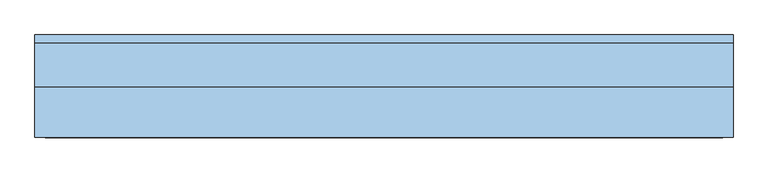
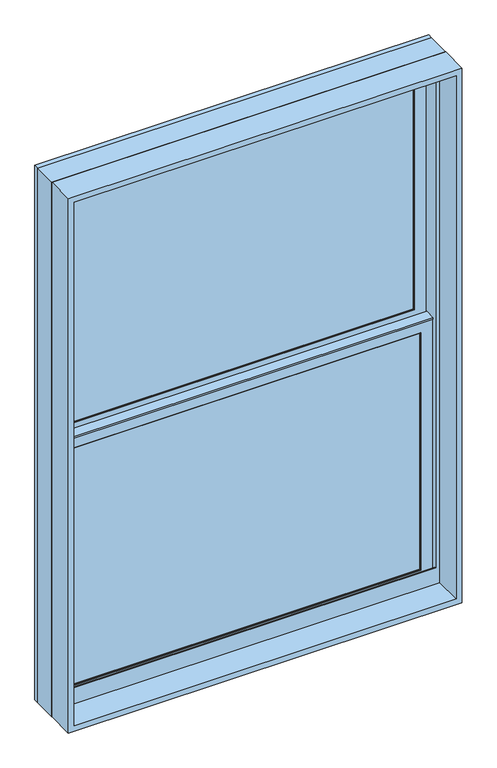
"""IFC4 building model written with IfcOpenShell, lengths in millimetres: window geometry, Window-Double_Hung-Marvin-Essential : ESDH3650."""

import ifcopenshell
import ifcopenshell.guid

model = None  # the IFC model being written
_history = None  # IfcOwnerHistory: only IFC2X3 demands one
_inside = {}  # id of a spatial element -> (the spatial element, [elements in it])
_under = {}  # id of a project, library or spatial element -> (it, [spatial elements below it])
_declared = {}  # id of a project -> (the project, [libraries it declares])
_typed = {}  # id of a type object -> (the type object, [elements of that type])
_made_of = {}  # id of a material, layer set ... -> (it, [elements and type objects made of it])


def new_model(schema):
    """Start an empty IFC model of exactly this schema.

    Asked for "IFC4X3", IfcOpenShell would pick the latest addendum, in which some entities
    have other attributes; the version numbers below select the first issue.
    IFC2X3 requires an IfcOwnerHistory on every rooted entity: one is made here for all.
    """
    global model, _history
    if schema == "IFC4X3":
        model = ifcopenshell.file(schema_version=(4, 3, 0, 0))
    else:
        model = ifcopenshell.file(schema=schema)
    _inside.clear()
    _under.clear()
    _declared.clear()
    _typed.clear()
    _made_of.clear()
    _history = None
    if model.schema == "IFC2X3":
        org = make("IfcOrganization", Name="unknown")
        user = make(
            "IfcPersonAndOrganization",
            ThePerson=make("IfcPerson", FamilyName="unknown"),
            TheOrganization=org,
        )
        app = make(
            "IfcApplication",
            ApplicationDeveloper=org,
            Version="unknown",
            ApplicationFullName="unknown",
            ApplicationIdentifier="unknown",
        )
        _history = make(
            "IfcOwnerHistory",
            OwningUser=user,
            OwningApplication=app,
            ChangeAction="ADDED",
            CreationDate=0,
        )
    return model


def make(cls, **values):
    """One entity of the class cls with the attributes given. An attribute that is None is left unset."""
    return model.create_entity(
        cls, **{name: value for name, value in values.items() if value is not None}
    )


def rooted(cls, **values):
    """An entity with a GlobalId (a new one), such as an element, a storey or a relation."""
    return make(cls, GlobalId=ifcopenshell.guid.new(), OwnerHistory=_history, **values)


def si_unit(unit_type, name, prefix=None):
    """IfcSIUnit, for example si_unit("LENGTHUNIT", "METRE", prefix="MILLI")."""
    return make("IfcSIUnit", UnitType=unit_type, Prefix=prefix, Name=name)


def assignment(units):
    """IfcUnitAssignment: the units of a project."""
    return None if units is None else make("IfcUnitAssignment", Units=units)


def point(xyz):
    """IfcCartesianPoint."""
    return None if xyz is None else make("IfcCartesianPoint", Coordinates=xyz)


def direction(xyz):
    """IfcDirection."""
    return None if xyz is None else make("IfcDirection", DirectionRatios=xyz)


def frame(location, z_axis=None, x_axis=None):
    """IfcAxis2Placement3D, a coordinate frame: its origin and axes. An axis left out is left unset."""
    return make(
        "IfcAxis2Placement3D",
        Location=point(location),
        Axis=direction(z_axis),
        RefDirection=direction(x_axis),
    )


def origin():
    """The frame at (0, 0, 0) with its axes left unset."""
    return frame((0.0, 0.0, 0.0))


def place(relative_to, where):
    """IfcLocalPlacement: puts the frame where relative to a parent placement (None: the world)."""
    return make(
        "IfcLocalPlacement", PlacementRelTo=relative_to, RelativePlacement=where
    )


def context(
    kind, dimensions, precision=None, world=None, true_north=None, identifier=None
):
    """IfcGeometricRepresentationContext, for example the 3D "Model" context."""
    return make(
        "IfcGeometricRepresentationContext",
        ContextIdentifier=identifier,
        ContextType=kind,
        CoordinateSpaceDimension=dimensions,
        Precision=precision,
        WorldCoordinateSystem=world,
        TrueNorth=true_north,
    )


def project(units=None, contexts=None):
    """IfcProject with its units and contexts."""
    return rooted(
        "IfcProject",
        Name="project",
        RepresentationContexts=contexts,
        UnitsInContext=assignment(units),
    )


def spatial(cls, under=None, at=None, **own):
    """A site, building, storey or space (cls), placed at a placement, below another one or the project."""
    s = rooted(cls, ObjectPlacement=at, **own)
    if under is not None:
        _under.setdefault(under.id(), (under, []))[1].append(s)
    return s


def polyline(points):
    """IfcPolyline through the points."""
    return make("IfcPolyline", Points=[point(p) for p in points])


def outline(outer, holes=None, kind="AREA"):
    """IfcArbitraryClosedProfileDef: a profile drawn as a closed curve; with holes, ...WithVoids."""
    if holes is None:
        return make("IfcArbitraryClosedProfileDef", ProfileType=kind, OuterCurve=outer)
    return make(
        "IfcArbitraryProfileDefWithVoids",
        ProfileType=kind,
        OuterCurve=outer,
        InnerCurves=holes,
    )


def extrude(swept, where, along, depth):
    """IfcExtrudedAreaSolid: the profile swept, set in the frame where, extruded along a direction by depth."""
    return make(
        "IfcExtrudedAreaSolid",
        SweptArea=swept,
        Position=where,
        ExtrudedDirection=direction(along),
        Depth=depth,
    )


def faces_of(points, faces, orient=None, outer=None):
    """IfcFace entities. A face is a list of loops; a loop is a list of indices into points, from 0.

    orient and outer hold one flag for each loop. By default every Orientation is true, the
    first loop of a face is its IfcFaceOuterBound and the others are IfcFaceBound.
    """
    made = []
    for i, loops in enumerate(faces):
        bounds = []
        for j, loop in enumerate(loops):
            is_outer = j == 0 if outer is None else outer[i][j]
            bounds.append(
                make(
                    "IfcFaceOuterBound" if is_outer else "IfcFaceBound",
                    Bound=make("IfcPolyLoop", Polygon=[points[k] for k in loop]),
                    Orientation=True if orient is None else orient[i][j],
                )
            )
        made.append(make("IfcFace", Bounds=bounds))
    return made


def faceted_brep(points, faces, orient=None, outer=None, voids=None):
    """IfcFacetedBrep: a solid bounded by flat faces; with voids (closed shells), ...WithVoids."""
    shared = [point(p) for p in points]
    hull = make("IfcClosedShell", CfsFaces=faces_of(shared, faces, orient, outer))
    if voids is None:
        return make("IfcFacetedBrep", Outer=hull)
    return make(
        "IfcFacetedBrepWithVoids",
        Outer=hull,
        Voids=[
            make(cls, CfsFaces=faces_of(shared, fs, o, b)) for cls, fs, o, b in voids
        ],
    )


def shape(context_of_items, identifier, shape_type, items):
    """IfcShapeRepresentation: the items that make up one representation, for example the "Body"."""
    return make(
        "IfcShapeRepresentation",
        ContextOfItems=context_of_items,
        RepresentationIdentifier=identifier,
        RepresentationType=shape_type,
        Items=items,
    )


def source(mapping_origin, context_of_items, identifier, shape_type, items):
    """IfcRepresentationMap: a shape defined once, which mapped items show again and again."""
    return make(
        "IfcRepresentationMap",
        MappingOrigin=mapping_origin,
        MappedRepresentation=shape(context_of_items, identifier, shape_type, items),
    )


def transform(
    local_origin,
    x_axis=None,
    y_axis=None,
    z_axis=None,
    scale=None,
    scale2=None,
    scale3=None,
    uniform=True,
):
    """IfcCartesianTransformationOperator3D, or its non-uniform kind. x_axis, y_axis, z_axis: its Axis1, 2, 3."""
    if uniform:
        return make(
            "IfcCartesianTransformationOperator3D",
            Axis1=direction(x_axis),
            Axis2=direction(y_axis),
            LocalOrigin=point(local_origin),
            Scale=scale,
            Axis3=direction(z_axis),
        )
    return make(
        "IfcCartesianTransformationOperator3DnonUniform",
        Axis1=direction(x_axis),
        Axis2=direction(y_axis),
        LocalOrigin=point(local_origin),
        Scale=scale,
        Axis3=direction(z_axis),
        Scale2=scale2,
        Scale3=scale3,
    )


def mapped(mapping_source, mapping_target):
    """IfcMappedItem: shows the shape of a source again, moved by a transform."""
    return make(
        "IfcMappedItem", MappingSource=mapping_source, MappingTarget=mapping_target
    )


def made_of(thing, what):
    """Note that an element or type object is made of a material, layer set ...; save() writes the relation."""
    if what is not None:
        _made_of.setdefault(what.id(), (what, []))[1].append(thing)
    return thing


def element(
    cls,
    number,
    at=None,
    inside=None,
    cuts=None,
    type_object=None,
    material=None,
    context=None,
    identifier="Body",
    shape_type=None,
    held_by="IfcProductDefinitionShape",
    body=None,
    shapes=None,
    **own,
):
    """One element of the class cls, such as IfcWall. Its Tag is "e" and its number.

    at: its placement. inside: the storey or other place that contains it. cuts: it is an
    opening in that element (IfcRelVoidsElement). A single representation is given by context,
    identifier, shape_type and body (its items); several are given by shapes. held_by: the class
    of the entity that holds the representations. save() writes the other relations.
    """
    e = rooted(cls, Tag="e%d" % number, ObjectPlacement=at, **own)
    if body is not None:
        shapes = [shape(context, identifier, shape_type, body)]
    if shapes is not None:
        e.Representation = make(held_by, Representations=shapes)
    if inside is not None:
        _inside.setdefault(inside.id(), (inside, []))[1].append(e)
    if cuts is not None:
        rooted(
            "IfcRelVoidsElement", RelatingBuildingElement=cuts, RelatedOpeningElement=e
        )
    if type_object is not None:
        _typed.setdefault(type_object.id(), (type_object, []))[1].append(e)
    return made_of(e, material)


def aggregate(whole, parts):
    """IfcRelAggregates: a whole, such as a stair, and the parts it consists of."""
    return rooted("IfcRelAggregates", RelatingObject=whole, RelatedObjects=parts)


def save(model, path):
    """Write the relations noted so far, then the file.

    IfcRelAggregates (storeys below a building ...), IfcRelContainedInSpatialStructure (elements
    in a storey), IfcRelDefinesByType, IfcRelAssociatesMaterial and IfcRelDeclares: one each for
    every whole, place, type object, material and project.
    """
    for whole, parts in _under.values():
        aggregate(whole, parts)
    for where, things in _inside.values():
        rooted(
            "IfcRelContainedInSpatialStructure",
            RelatedElements=things,
            RelatingStructure=where,
        )
    for kind, things in _typed.values():
        rooted("IfcRelDefinesByType", RelatedObjects=things, RelatingType=kind)
    for what, things in _made_of.values():
        rooted("IfcRelAssociatesMaterial", RelatedObjects=things, RelatingMaterial=what)
    for by, libraries in _declared.values():
        rooted("IfcRelDeclares", RelatingContext=by, RelatedDefinitions=libraries)
    model.write(path)


def window_911fa5ce(model_context):
    return source(origin(), model_context, "Body", "SolidModel", [
        extrude(outline(polyline([(166.1583333, 20.6375), (166.1583333, 15.875), (147.1083333, 15.875), (147.1083333, 20.6375), (166.1583333, 20.6375)])), frame((0.0, 0.0, 984.25), z_axis=(0.0, 0.0, 1.0), x_axis=(1.0, 0.0, 0.0)), (0.0, 0.0, 1.0), 679.45),
        extrude(outline(polyline([(-147.1083333, 20.6375), (-147.1083333, 15.875), (-166.1583333, 15.875), (-166.1583333, 20.6375), (-147.1083333, 20.6375)])), frame((0.0, 0.0, 984.25), z_axis=(0.0, 0.0, 1.0), x_axis=(1.0, 0.0, 0.0)), (0.0, 0.0, 1.0), 679.45),
        extrude(outline(polyline([(469.9, 20.6375), (469.9, 15.875), (-469.9, 15.875), (-469.9, 20.6375), (469.9, 20.6375)])), frame((0.0, 0.0, 1314.45), z_axis=(0.0, 0.0, 1.0), x_axis=(1.0, 0.0, 0.0)), (0.0, 0.0, 1.0), 19.05),
        extrude(outline(polyline([(-166.1583333, 46.83125), (-166.1583333, 51.59375), (-147.1083333, 51.59375), (-147.1083333, 46.83125), (-166.1583333, 46.83125)])), frame((0.0, 0.0, 1701.8), z_axis=(0.0, 0.0, 1.0), x_axis=(1.0, 0.0, 0.0)), (0.0, 0.0, 1.0), 679.45),
        extrude(outline(polyline([(147.1083333, 46.83125), (147.1083333, 51.59375), (166.1583333, 51.59375), (166.1583333, 46.83125), (147.1083333, 46.83125)])), frame((0.0, 0.0, 1701.8), z_axis=(0.0, 0.0, 1.0), x_axis=(1.0, 0.0, 0.0)), (0.0, 0.0, 1.0), 679.45),
        extrude(outline(polyline([(-469.9, 46.83125), (-469.9, 51.59375), (469.9, 51.59375), (469.9, 46.83125), (-469.9, 46.83125)])), frame((0.0, 0.0, 2032.0), z_axis=(0.0, 0.0, 1.0), x_axis=(1.0, 0.0, 0.0)), (0.0, 0.0, 1.0), 19.05),
        extrude(outline(polyline([(166.1583333, 20.6375), (147.1083333, 20.6375), (147.1083333, 25.4), (166.1583333, 25.4), (166.1583333, 20.6375)])), frame((0.0, 0.0, 984.25), z_axis=(0.0, 0.0, 1.0), x_axis=(1.0, 0.0, 0.0)), (0.0, 0.0, 1.0), 679.45),
        extrude(outline(polyline([(-147.1083333, 20.6375), (-166.1583333, 20.6375), (-166.1583333, 25.4), (-147.1083333, 25.4), (-147.1083333, 20.6375)])), frame((0.0, 0.0, 984.25), z_axis=(0.0, 0.0, 1.0), x_axis=(1.0, 0.0, 0.0)), (0.0, 0.0, 1.0), 679.45),
        extrude(outline(polyline([(469.9, 20.6375), (-469.9, 20.6375), (-469.9, 25.4), (469.9, 25.4), (469.9, 20.6375)])), frame((0.0, 0.0, 1314.45), z_axis=(0.0, 0.0, 1.0), x_axis=(1.0, 0.0, 0.0)), (0.0, 0.0, 1.0), 19.05),
        extrude(outline(polyline([(-166.1583333, 56.35625), (-147.1083333, 56.35625), (-147.1083333, 51.59375), (-166.1583333, 51.59375), (-166.1583333, 56.35625)])), frame((0.0, 0.0, 1701.8), z_axis=(0.0, 0.0, 1.0), x_axis=(1.0, 0.0, 0.0)), (0.0, 0.0, 1.0), 679.45),
        extrude(outline(polyline([(147.1083333, 56.35625), (166.1583333, 56.35625), (166.1583333, 51.59375), (147.1083333, 51.59375), (147.1083333, 56.35625)])), frame((0.0, 0.0, 1701.8), z_axis=(0.0, 0.0, 1.0), x_axis=(1.0, 0.0, 0.0)), (0.0, 0.0, 1.0), 679.45),
        extrude(outline(polyline([(-469.9, 56.35625), (469.9, 56.35625), (469.9, 51.59375), (-469.9, 51.59375), (-469.9, 56.35625)])), frame((0.0, 0.0, 2032.0), z_axis=(0.0, 0.0, 1.0), x_axis=(1.0, 0.0, 0.0)), (0.0, 0.0, 1.0), 19.05),
        faceted_brep([(-496.8875, 5.6780605, 1693.7351748), (-496.8875, 5.6780605, 1689.1), (496.8875, 5.6780605, 1689.1), (496.8875, 5.6780605, 1693.7351748), (-496.8875, 34.8118605, 1693.7351748), (496.8875, 34.8118605, 1693.7351748), (496.8875, 34.8118605, 1689.1), (-496.8875, 34.8118605, 1689.1), (-496.8875, 30.1625, 1689.1), (-496.8875, 30.1625, 957.2625), (-496.8875, 8.9241104, 957.2625), (-496.8875, 8.9241104, 1689.1), (496.8875, 8.9241104, 1689.1), (496.8875, 30.1625, 1689.1), (496.8875, 8.9241104, 957.2625), (496.8875, 30.1625, 957.2625), (-481.0034752, 11.90625, 1674.8034752), (-481.0034752, 30.1625, 1674.8034752), (481.0034752, 30.1625, 1674.8034752), (481.0034752, 11.90625, 1674.8034752), (-464.34375, 10.4662439, 1658.14375), (-464.34375, 11.90625, 1658.14375), (464.34375, 11.90625, 1658.14375), (464.34375, 10.4662439, 1658.14375), (465.8858834, 8.9241104, 1659.6858834), (-465.8858834, 8.9241104, 1659.6858834), (481.0034752, 30.1625, 973.1465248), (481.0034752, 11.90625, 973.1465248), (464.34375, 11.90625, 989.80625), (464.34375, 10.4662439, 989.80625), (465.8858834, 8.9241104, 988.2641166), (-481.0034752, 30.1625, 973.1465248), (-481.0034752, 11.90625, 973.1465248), (-464.34375, 11.90625, 989.80625), (-464.34375, 10.4662439, 989.80625), (-465.8858834, 8.9241104, 988.2641166)], [[[0, 1, 2, 3]], [[4, 5, 6, 7]], [[1, 0, 4, 7, 8, 9, 10, 11]], [[2, 1, 11, 12]], [[7, 6, 13, 8]], [[3, 2, 12, 14, 15, 13, 6, 5]], [[0, 3, 5, 4]], [[16, 17, 18, 19]], [[20, 21, 22, 23]], [[20, 23, 24, 25]], [[19, 18, 26, 27]], [[23, 22, 28, 29]], [[24, 23, 29, 30]], [[27, 26, 31, 32]], [[29, 28, 33, 34]], [[30, 29, 34, 35]], [[15, 14, 10, 9]], [[15, 9, 8, 13], [18, 17, 31, 26]], [[17, 16, 32, 31]], [[16, 19, 27, 32], [22, 21, 33, 28]], [[21, 20, 34, 33]], [[20, 25, 35, 34]], [[10, 14, 12, 11], [25, 24, 30, 35]]]),
        extrude(outline(polyline([(38.5955581, 1674.8125), (33.5778968, 1674.8125), (33.5778968, 1676.4), (39.9405976, 1676.4), (39.9405976, 1674.8125), (61.515625, 1674.8125), (47.6307501, 1671.4975159), (38.5955581, 1671.4975159), (38.5955581, 1674.8125)])), frame((-496.8875, 0.0, 0.0), z_axis=(1.0, 0.0, 0.0), x_axis=(0.0, 1.0, 0.0)), (0.0, 0.0, 1.0), 993.775),
        faceted_brep([(527.05, 0.0, 927.1), (527.05, 0.0, 2438.4), (-527.05, 0.0, 2438.4), (-527.05, 0.0, 927.1), (500.85625, 0.0, 988.21875), (-500.85625, 0.0, 988.21875), (-500.85625, 0.0, 2412.20625), (500.85625, 0.0, 2412.20625), (500.85625, 3.96875, 927.1), (-500.85625, 3.96875, 927.1), (-500.85625, 3.96875, 988.21875), (500.85625, 3.96875, 988.21875), (-527.05, 65.6828125, 927.1), (-500.85625, 65.6828125, 927.1), (500.85625, 65.6828125, 927.1), (527.05, 65.6828125, 927.1), (-527.05, 65.6828125, 2438.4), (527.05, 65.6828125, 2438.4), (500.85625, 65.6828125, 2412.20625), (-500.85625, 65.6828125, 2412.20625)], [[[0, 1, 2, 3], [4, 5, 6, 7]], [[8, 9, 10, 11]], [[5, 4, 11, 10]], [[0, 3, 12, 13, 9, 8, 14, 15]], [[13, 12, 16, 17, 15, 14, 18, 19]], [[13, 19, 6, 5, 10, 9]], [[7, 6, 19, 18]], [[18, 14, 8, 11, 4, 7]], [[1, 0, 15, 17]], [[2, 1, 17, 16]], [[3, 2, 16, 12]]]),
        faceted_brep([(500.85625, 30.1625, 1682.75), (499.26875, 30.1625, 1682.75), (499.26875, 30.1625, 951.4544613), (500.85625, 30.1625, 951.4544613), (-499.26875, 30.1625, 1682.75), (-500.85625, 30.1625, 1682.75), (-500.85625, 30.1625, 951.4544613), (-499.26875, 30.1625, 951.4544613), (499.26875, 63.5, 1682.75), (500.85625, 63.5, 1682.75), (500.85625, 63.5, 944.9743077), (499.26875, 63.5, 944.9743077), (-500.85625, 63.5, 1682.75), (-499.26875, 63.5, 1682.75), (-499.26875, 63.5, 944.9743077), (-500.85625, 63.5, 944.9743077), (512.1108932, 3.96875, 956.5460105), (512.1108932, 3.96875, 927.1), (512.1108932, 65.6828125, 927.1), (512.1108932, 65.6828125, 944.550012), (-512.1108932, 3.96875, 927.1), (-512.1108932, 3.96875, 956.5460105), (-512.1108932, 65.6828125, 944.550012), (-512.1108932, 65.6828125, 927.1), (512.1108932, 78.58125, 942.0428097), (-512.1108932, 78.58125, 942.0428097), (-510.0971252, 68.2348864, 944.0539391), (-492.13135, 68.2348864, 944.0539391), (-492.13135, 65.6828125, 944.550012), (492.13135, 65.6828125, 944.550012), (492.13135, 68.2348864, 944.0539391), (510.0971252, 68.2348864, 944.0539391), (-527.05, 65.6828125, 927.1), (-527.05, 78.5948249, 927.1), (527.05, 78.5948249, 927.1), (527.05, 65.6828125, 927.1), (-527.05, 78.58125, 2438.4), (527.05, 78.58125, 2438.4), (512.1108932, 78.58125, 2423.4608932), (-512.1108932, 78.58125, 2423.4608932), (-527.05, 65.6828125, 2438.4), (-510.0971252, 68.2348864, 2421.4471252), (510.0971252, 68.2348864, 2421.4471252), (492.13135, 68.2348864, 2403.48135), (-492.13135, 68.2348864, 2403.48135), (-492.13135, 65.6828125, 2403.48135), (492.13135, 65.6828125, 2403.48135), (527.05, 65.6828125, 2438.4)], [[[0, 1, 2, 3]], [[4, 5, 6, 7]], [[8, 9, 10, 11]], [[12, 13, 14, 15]], [[1, 8, 11, 2]], [[9, 0, 3, 10]], [[1, 0, 9, 8]], [[5, 4, 13, 12]], [[5, 12, 15, 6]], [[13, 4, 7, 14]], [[16, 17, 18, 19]], [[20, 21, 22, 23]], [[24, 25, 26, 27, 28, 22, 21, 16, 19, 29, 30, 31], [3, 2, 11, 10], [7, 6, 15, 14]], [[17, 16, 21, 20]], [[17, 20, 23, 32, 33, 34, 35, 18]], [[34, 33, 36, 37], [25, 24, 38, 39]], [[33, 32, 40, 36]], [[39, 41, 26, 25]], [[41, 42, 31, 30, 43, 44, 27, 26]], [[44, 45, 28, 27]], [[40, 32, 23, 22, 28, 45, 46, 29, 19, 18, 35, 47]], [[36, 40, 47, 37]], [[39, 38, 42, 41]], [[44, 43, 46, 45]], [[34, 37, 47, 35]], [[42, 38, 24, 31]], [[46, 43, 30, 29]]]),
        extrude(outline(polyline([(477.04375, 11.90625), (-477.04375, 11.90625), (-477.04375, 15.08125), (477.04375, 15.08125), (477.04375, 11.90625)])), frame((0.0, 0.0, 977.10625), z_axis=(0.0, 0.0, 1.0), x_axis=(1.0, 0.0, 0.0)), (0.0, 0.0, 1.0), 693.7375),
        extrude(outline(polyline([(477.04375, 42.8625), (-477.04375, 42.8625), (-477.04375, 46.0375), (477.04375, 46.0375), (477.04375, 42.8625)])), frame((0.0, 0.0, 1694.65625), z_axis=(0.0, 0.0, 1.0), x_axis=(1.0, 0.0, 0.0)), (0.0, 0.0, 1.0), 693.7375),
        faceted_brep([(-464.34375, 31.194477, 1658.14375), (-465.8858834, 32.7366104, 1659.6858834), (465.8858834, 32.7366104, 1659.6858834), (464.34375, 31.194477, 1658.14375), (-464.34375, 30.1625, 1658.14375), (464.34375, 30.1625, 1658.14375), (-496.8875, 32.7366104, 1690.6875), (-496.8875, 30.1625, 1690.6875), (496.8875, 30.1625, 1690.6875), (496.8875, 32.7366104, 1690.6875), (465.8858834, 32.7366104, 988.2641166), (464.34375, 31.194477, 989.80625), (464.34375, 30.1625, 989.80625), (496.8875, 30.1625, 957.2625), (496.8875, 32.7366104, 957.2625), (-465.8858834, 32.7366104, 988.2641166), (-464.34375, 31.194477, 989.80625), (-464.34375, 30.1625, 989.80625), (-496.8875, 30.1625, 957.2625), (-496.8875, 32.7366104, 957.2625)], [[[0, 1, 2, 3]], [[4, 0, 3, 5]], [[6, 7, 8, 9]], [[3, 2, 10, 11]], [[5, 3, 11, 12]], [[9, 8, 13, 14]], [[11, 10, 15, 16]], [[12, 11, 16, 17]], [[14, 13, 18, 19]], [[9, 14, 19, 6], [1, 15, 10, 2]], [[16, 15, 1, 0]], [[17, 16, 0, 4]], [[7, 18, 13, 8], [5, 12, 17, 4]], [[19, 18, 7, 6]]]),
        faceted_brep([(-481.0034752, 42.8625, 2392.3534752), (-481.0034752, 61.11875, 2392.3534752), (481.0034752, 61.11875, 2392.3534752), (481.0034752, 42.8625, 2392.3534752), (-464.34375, 41.4224939, 2375.69375), (-464.34375, 42.8625, 2375.69375), (464.34375, 42.8625, 2375.69375), (464.34375, 41.4224939, 2375.69375), (-465.8858834, 39.8803604, 2377.2358834), (465.8858834, 39.8803604, 2377.2358834), (-496.8875, 61.11875, 2408.2375), (-496.8875, 39.8803604, 2408.2375), (496.8875, 39.8803604, 2408.2375), (496.8875, 61.11875, 2408.2375), (481.0034752, 61.11875, 1690.6965248), (481.0034752, 42.8625, 1690.6965248), (464.34375, 42.8625, 1707.35625), (464.34375, 41.4224939, 1707.35625), (465.8858834, 39.8803604, 1705.8141166), (496.8875, 39.8803604, 1674.8125), (496.8875, 61.11875, 1674.8125), (-481.0034752, 61.11875, 1690.6965248), (-481.0034752, 42.8625, 1690.6965248), (-464.34375, 42.8625, 1707.35625), (-464.34375, 41.4224939, 1707.35625), (-465.8858834, 39.8803604, 1705.8141166), (-496.8875, 39.8803604, 1674.8125), (-496.8875, 61.11875, 1674.8125)], [[[0, 1, 2, 3]], [[4, 5, 6, 7]], [[8, 4, 7, 9]], [[10, 11, 12, 13]], [[3, 2, 14, 15]], [[7, 6, 16, 17]], [[9, 7, 17, 18]], [[13, 12, 19, 20]], [[15, 14, 21, 22]], [[17, 16, 23, 24]], [[18, 17, 24, 25]], [[20, 19, 26, 27]], [[13, 20, 27, 10], [1, 21, 14, 2]], [[22, 21, 1, 0]], [[3, 15, 22, 0], [5, 23, 16, 6]], [[24, 23, 5, 4]], [[25, 24, 4, 8]], [[11, 26, 19, 12], [9, 18, 25, 8]], [[27, 26, 11, 10]]]),
        faceted_brep([(-496.8875, 61.11875, 1674.8125), (-496.8875, 63.6928604, 1674.8125), (496.8875, 63.6928604, 1674.8125), (496.8875, 61.11875, 1674.8125), (-464.34375, 62.150727, 1707.35625), (-464.34375, 61.11875, 1707.35625), (464.34375, 61.11875, 1707.35625), (464.34375, 62.150727, 1707.35625), (-465.8858834, 63.6928604, 1705.8141166), (465.8858834, 63.6928604, 1705.8141166), (496.8875, 63.6928604, 2408.2375), (496.8875, 61.11875, 2408.2375), (464.34375, 61.11875, 2375.69375), (464.34375, 62.150727, 2375.69375), (465.8858834, 63.6928604, 2377.2358834), (-496.8875, 63.6928604, 2408.2375), (-496.8875, 61.11875, 2408.2375), (-464.34375, 61.11875, 2375.69375), (-464.34375, 62.150727, 2375.69375), (-465.8858834, 63.6928604, 2377.2358834)], [[[0, 1, 2, 3]], [[4, 5, 6, 7]], [[8, 4, 7, 9]], [[3, 2, 10, 11]], [[7, 6, 12, 13]], [[9, 7, 13, 14]], [[11, 10, 15, 16]], [[13, 12, 17, 18]], [[14, 13, 18, 19]], [[16, 15, 1, 0]], [[3, 11, 16, 0], [5, 17, 12, 6]], [[18, 17, 5, 4]], [[19, 18, 4, 8]], [[1, 15, 10, 2], [9, 14, 19, 8]]]),
        extrude(outline(polyline([(477.04375, 26.19375), (-477.04375, 26.19375), (-477.04375, 30.1625), (477.04375, 30.1625), (477.04375, 26.19375)])), frame((0.0, 0.0, 977.10625), z_axis=(0.0, 0.0, 1.0), x_axis=(1.0, 0.0, 0.0)), (0.0, 0.0, 1.0), 693.7375),
        extrude(outline(polyline([(477.04375, 57.15), (-477.04375, 57.15), (-477.04375, 61.11875), (477.04375, 61.11875), (477.04375, 57.15)])), frame((0.0, 0.0, 1694.65625), z_axis=(0.0, 0.0, 1.0), x_axis=(1.0, 0.0, 0.0)), (0.0, 0.0, 1.0), 693.7375),
        extrude(outline(polyline([(2438.4, 527.05), (2438.4, -527.05), (927.1, -527.05), (927.1, 527.05), (2438.4, 527.05)]), holes=[polyline([(2422.525, 511.175), (942.975, 511.175), (942.975, -511.175), (2422.525, -511.175), (2422.525, 511.175)])]), frame((0.0, -76.2, 0.0), z_axis=(0.0, 1.0, 0.0), x_axis=(0.0, 0.0, 1.0)), (0.0, 0.0, 1.0), 75.40625),
    ])


if __name__ == "__main__":
    model = new_model("IFC4")
    model_context = context("Model", 3, world=origin())
    ifc_project = project(units=[si_unit("LENGTHUNIT", "METRE", prefix="MILLI")], contexts=[model_context])
    site = spatial("IfcSite", under=ifc_project)
    building = spatial("IfcBuilding", under=site)
    placement = place(None, origin())
    window_shape = window_911fa5ce(model_context)
    element("IfcWindow", 1, ObjectType="Window-Double_Hung-Marvin-Essential : ESDH3650", at=placement, inside=building, context=model_context, shape_type="MappedRepresentation", body=[
        mapped(window_shape, transform((0.0, 0.0, 0.0), x_axis=(1.0, 0.0, 0.0), y_axis=(0.0, 1.0, 0.0), z_axis=(0.0, 0.0, 1.0))),
    ])
    save(model, "model.ifc")

# Revit data of these elements
# Type "Window-Double_Hung-Marvin-Essential : ESDH3650"
#   Type Mark = "66"
#   Window Type = "Essential Double Hung"
#   Product data url = "https://bimobject.com/marvin-windows-and-doors/product/marvin-dhwau"
#   Product Guid = "c4a96547-874c-4385-91dc-a058adc19d98"
#   Frame = "All Ultrex"
#   Egress Window = "Yes"
#   URL = "www.marvin.com"
#   Model = "ESDH3650"
#   Manufacturer = "Marvin Windows and Doors"
#   Label Egress = "EGRESS WDW"
#   Glass Type = "IG Low E II with Argon"
#   Design Pressure = "DP40"
#   Description = "4260 DBHG"
#   Analytic Construction = "<None>"
#   Prairie Corner Width = 0' - 4"
#   Prairie Corner Height = 0' - 4"
#   Egress Width = 3' - 2 9/16"
#   Egress Height = 2' - 1 27/128"
#   Rough Width = 3' - 6"
#   Rough Height = 5' - 0"
#   Nominal Width = 3' - 6"
#   Nominal Height = 5' - 0"
#   Inset to Installation Flange [instance default] = 0' - 1"
#   Height = 4' - 11 1/2"
#   Egress Area = 6.75137 SF
#   Default Head Height = 8' - 0"
#   Width = 3' - 5 1/2"
#   Daylight Area = 13.3618 SF
#   DLO Width = 3' - 0 9/16"
#   DLO Height = 2' - 2 5/16"
#   Muntins Top Sash = yes
#   Lites Wide Top Sash = 3
#   Lites Wide Bottom Sash = 3
#   Lites High Top Sash = 2
#   Lites High Bottom Sash = 2
#   Lite Cut Prairie 9 = no
#   Lite Cut HV Grid = yes
#   Muntins Bottom Sash = yes
#   Label Visibility = no
#   Jamb Extension Visibility = yes
#   Edition number = 1
#   Interior Material = Ultrex-Marvin-Stonewhite
#   Glazing Material = Glass-Marvin-IG Low E II with Argon
#   Cladding Material = Ultrex-Marvin-Pebblegray
#   Wall Closure = (empty or 0)
#   Assembly Code = ""
# Element 1 (IfcWindow, "Window-Double_Hung-Marvin-Essential : ESDH3650")
#   Materials on its faces: "Ultrex-Marvin-Pebblegray", "Ultrex-Marvin-Stonewhite", "Glass-Marvin-IG Low E II with Argon"
# Materials
#   "Ultrex-Marvin-Stonewhite": class "Paint", colour RGB 250 251 245, transparency 0
#   "Glass-Marvin-IG Low E II with Argon": class "Glass", colour RGB 0 128 192, transparency 0.85
#   "Ultrex-Marvin-Pebblegray": class "Paint", colour RGB 189 185 173, transparency 0
